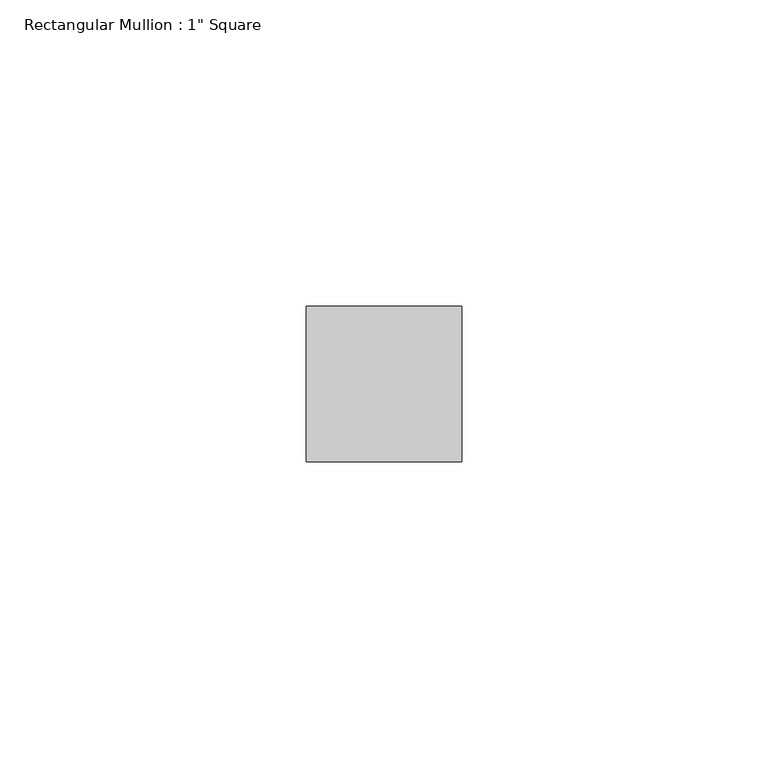
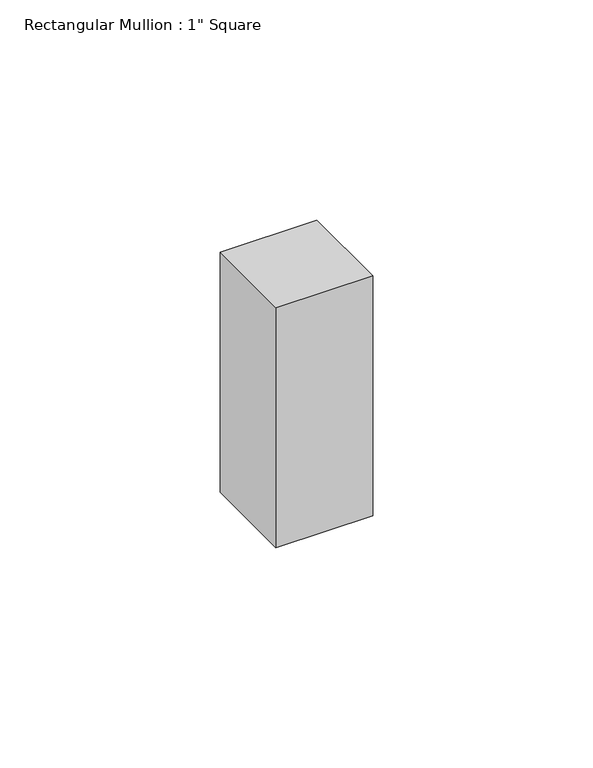
"""IFC4 building model written with IfcOpenShell, lengths in millimetres: member geometry."""

from ifc_helpers import new_model, si_unit, frame, origin, place, context, project, spatial, polyline, outline, extrude, source, transform, mapped, element, save


def member_be6bf66a(model_context):
    return source(origin(), model_context, "Body", "SweptSolid", [
        extrude(outline(polyline([(0.0, 12.7), (0.0, -12.7), (-25.4, -12.7), (-25.4, 12.7), (0.0, 12.7)])), frame((0.0, 0.0, -66.675), z_axis=(0.0, 0.0, 1.0), x_axis=(1.0, 0.0, 0.0)), (0.0, 0.0, 1.0), 66.675),
    ])


if __name__ == "__main__":
    model = new_model("IFC4")
    model_context = context("Model", 3, world=origin())
    ifc_project = project(units=[si_unit("LENGTHUNIT", "METRE", prefix="MILLI")], contexts=[model_context])
    site = spatial("IfcSite", under=ifc_project)
    building = spatial("IfcBuilding", under=site)
    placement = place(None, origin())
    member_shape = member_be6bf66a(model_context)
    element("IfcMember", 1, ObjectType="Rectangular Mullion : 1\" Square", at=placement, inside=building, context=model_context, shape_type="MappedRepresentation", body=[
        mapped(member_shape, transform((0.0, 0.0, 0.0), x_axis=(1.0, 0.0, 0.0), y_axis=(0.0, 1.0, 0.0), z_axis=(0.0, 0.0, 1.0))),
    ])
    save(model, "model.ifc")

# Revit data of these elements
# Type "Rectangular Mullion : 1\" Square"
#   built-in parameter 1007304 = 0.0833333 (stored number, unit not read)
#   built-in parameter 1007301 = 0.0416667 (stored number, unit not read)
#   built-in parameter 1007300 = 0.0416667 (stored number, unit not read)
# Element 1 (IfcMember, "Rectangular Mullion : 1\" Square")
#   Materials on its faces: "Metal - Aluminum"
# Materials
#   "Metal - Aluminum": class "Metal", colour RGB 247 247 247, transparency 0
